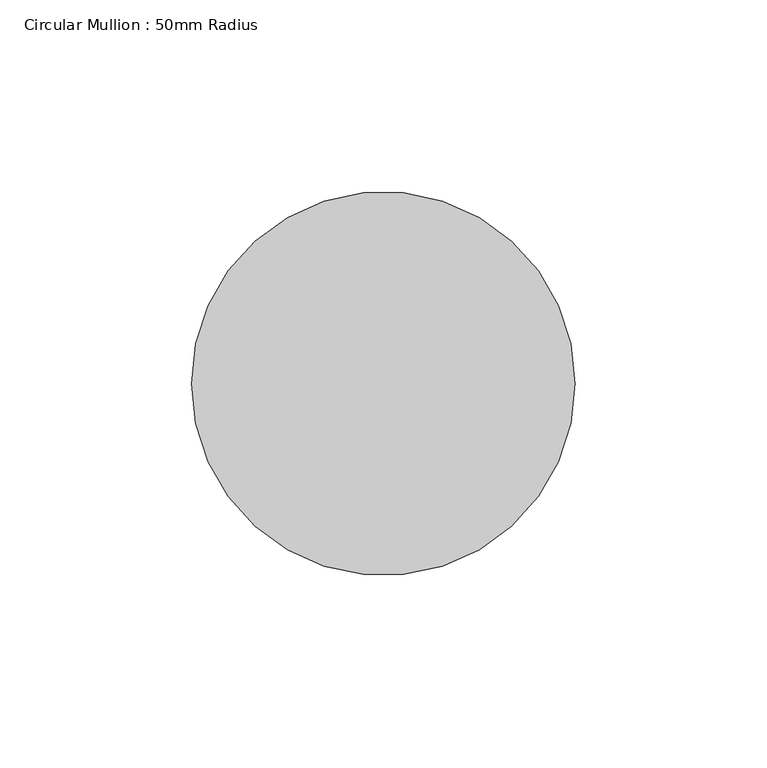
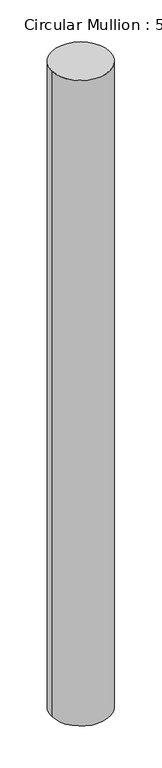
"""IFC4 building model written with IfcOpenShell, lengths in millimetres: member geometry, Circular Mullion : 50mm Radius."""

from ifc_helpers import new_model, si_unit, point, frame, origin, origin_2d, place, context, project, spatial, circle_curve, trimmed, segment, composite_curve, outline, extrude, source, transform, mapped, element, save


def circular_mullion_50mm_radius_6021110e(model_context):
    return source(origin(), model_context, "Body", "SweptSolid", [
        extrude(outline(composite_curve([segment(trimmed(circle_curve(origin_2d(), 50.0), [point((50.0, 0.0))], [point((-50.0, 0.0))], False, "CARTESIAN"), True, "CONTINUOUS"), segment(trimmed(circle_curve(origin_2d(), 50.0), [point((-50.0, 0.0))], [point((50.0, 0.0))], False, "CARTESIAN"), True, "CONTINUOUS")], self_intersect=False)), frame((0.0, 0.0, -1172.9140992), z_axis=(0.0, 0.0, 1.0), x_axis=(1.0, 0.0, 0.0)), (0.0, 0.0, 1.0), 1172.9140992),
    ])


if __name__ == "__main__":
    model = new_model("IFC4")
    model_context = context("Model", 3, world=origin())
    ifc_project = project(units=[si_unit("LENGTHUNIT", "METRE", prefix="MILLI")], contexts=[model_context])
    site = spatial("IfcSite", under=ifc_project)
    building = spatial("IfcBuilding", under=site)
    placement = place(None, origin())
    circular_mullion_50mm_radius_shape = circular_mullion_50mm_radius_6021110e(model_context)
    element("IfcMember", 1, ObjectType="Circular Mullion : 50mm Radius", at=placement, inside=building, context=model_context, shape_type="MappedRepresentation", body=[
        mapped(circular_mullion_50mm_radius_shape, transform((0.0, 0.0, 0.0), x_axis=(1.0, 0.0, 0.0), y_axis=(0.0, 1.0, 0.0), z_axis=(0.0, 0.0, 1.0))),
    ])
    save(model, "model.ifc")

# Revit data of these elements
# Type "Circular Mullion : 50mm Radius"
#   built-in parameter 1007350 = 0.164042 (stored number, unit not read)
# Element 1 (IfcMember, "Circular Mullion : 50mm Radius")
#   Materials on its faces: "Aluminium"
# Materials
#   "Aluminium": class "Metal", colour RGB 247 247 247, transparency 0, Description = "Aluminium 6061", Cost = 0
